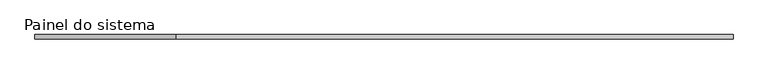
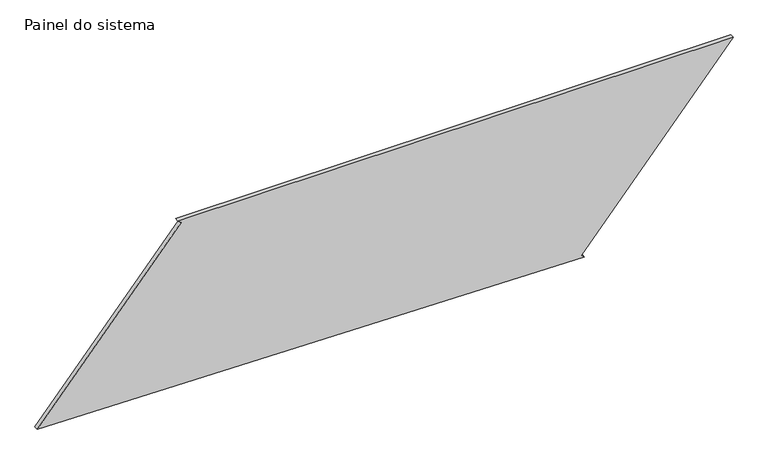
"""IFC4 building model written with IfcOpenShell, lengths in millimetres: plate geometry, Painel do sistema : Envidraçado."""

from ifc_helpers import new_model, si_unit, frame, origin, place, context, project, spatial, polyline, outline, extrude, source, transform, mapped, element, save


def painel_do_sistema_ccdc766c(model_context):
    return source(origin(), model_context, "Body", "SweptSolid", [
        extrude(outline(polyline([(0.0, 1202.1727359), (16.2242617, 1183.1523959), (1089.4544295, 2098.6127496), (1089.4544295, -1249.9458799), (1073.2301678, -1230.92554), (56.0063352, -2098.6127496), (0.0, 1202.1727359)])), frame((0.0, 24.5, 0.0), z_axis=(0.0, 1.0, 0.0), x_axis=(0.0, 0.0, 1.0)), (0.0, 0.0, 1.0), 25.0),
    ])


if __name__ == "__main__":
    model = new_model("IFC4")
    model_context = context("Model", 3, world=origin())
    ifc_project = project(units=[si_unit("LENGTHUNIT", "METRE", prefix="MILLI")], contexts=[model_context])
    site = spatial("IfcSite", under=ifc_project)
    building = spatial("IfcBuilding", under=site)
    placement = place(None, origin())
    painel_do_sistema_shape = painel_do_sistema_ccdc766c(model_context)
    element("IfcPlate", 1, ObjectType="Painel do sistema : Envidraçado", at=placement, inside=building, context=model_context, shape_type="MappedRepresentation", body=[
        mapped(painel_do_sistema_shape, transform((0.0, 0.0, 0.0), x_axis=(1.0, 0.0, 0.0), y_axis=(0.0, 1.0, 0.0), z_axis=(0.0, 0.0, 1.0))),
    ])
    save(model, "model.ifc")

# Revit data of these elements
# Type "Painel do sistema : Envidraçado"
#   Construction Type Id = "GSP4R"
#   Analytic Construction = "Vidraça única Pilkington 1/8 pol"
#   Visual Light Transmittance = 0.9
#   Solar Heat Gain Coefficient = 0.86
#   Heat Transfer Coefficient (U) = 6.7069 W/(m²·K)
# Element 1 (IfcPlate, "Painel do sistema : Envidraçado")
#   Materials on its faces: "Vidro"
# Materials
#   "Vidro": class "Vidro", colour RGB 0 128 192, transparency 0.9, Description = "Vidro de sílica", Cost = 0
